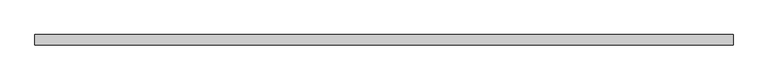
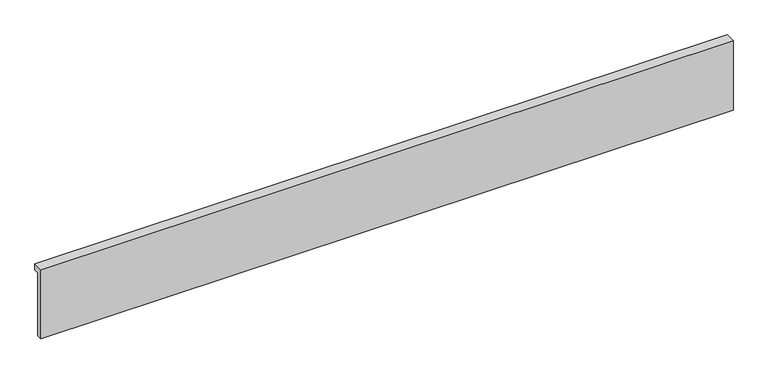
"""IFC4 building model written with IfcOpenShell, lengths in millimetres: proxy geometry, Stucco009 2225 : Stucco009 2225."""

from ifc_helpers import new_model, si_unit, frame, origin, place, context, project, spatial, polyline, outline, extrude, source, transform, mapped, element, save


def generic_models_48d159d9(model_context):
    return source(origin(), model_context, "Body", "SweptSolid", [
        extrude(outline(polyline([(9759.128362, 39738.0469041), (9789.2215225, 39738.0469041), (9789.2215225, 39718.9969041), (9774.9664479, 39718.9969041), (9774.9664479, 39526.5359375), (9759.128362, 39526.5359375), (9759.128362, 39738.0469041)])), frame((3694.2883192, 0.0, 0.0), z_axis=(1.0, 0.0, 0.0), x_axis=(0.0, 1.0, 0.0)), (0.0, 0.0, 1.0), 2000.0),
    ])


if __name__ == "__main__":
    model = new_model("IFC4")
    model_context = context("Model", 3, world=origin())
    ifc_project = project(units=[si_unit("LENGTHUNIT", "METRE", prefix="MILLI")], contexts=[model_context])
    site = spatial("IfcSite", under=ifc_project)
    building = spatial("IfcBuilding", under=site)
    placement = place(None, origin())
    generic_models_shape = generic_models_48d159d9(model_context)
    element("IfcBuildingElementProxy", 1, Name="Stucco009 2225 : Stucco009 2225", ObjectType="Stucco009 2225 : Stucco009 2225", at=placement, inside=building, context=model_context, shape_type="MappedRepresentation", body=[
        mapped(generic_models_shape, transform((0.0, 0.0, 0.0), x_axis=(1.0, 0.0, 0.0), y_axis=(0.0, 1.0, 0.0), z_axis=(0.0, 0.0, 1.0))),
    ])
    save(model, "model.ifc")

# Revit data of these elements
# Type "Stucco009 2225 : Stucco009 2225"
#   NameOverride = "Stucco009"
# Element 1 (IfcBuildingElementProxy, "Stucco009 2225 : Stucco009 2225")
#   Materials on its faces: "7/8\" SMOOTH TROWEL EXTERIOR STUCCO"
# Materials
#   "7/8\" SMOOTH TROWEL EXTERIOR STUCCO": class "Unassigned", colour RGB 255 255 255, transparency 0, Cost = 0
